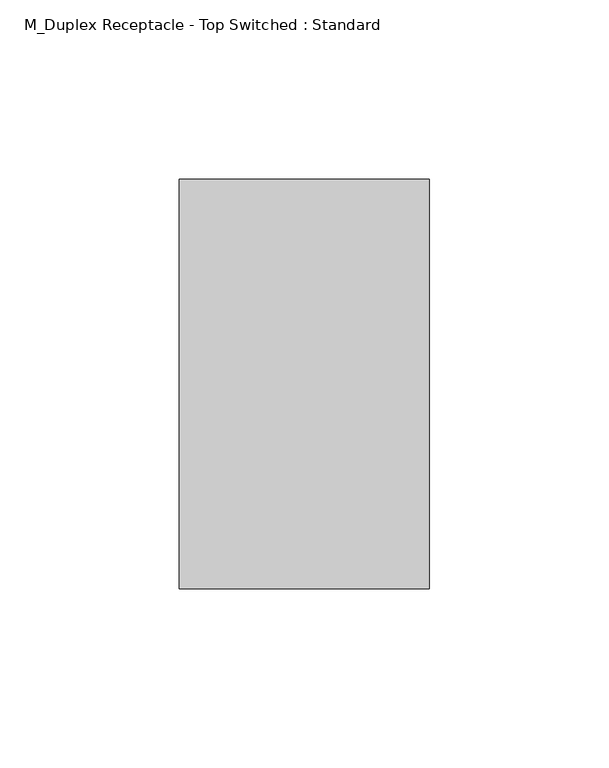
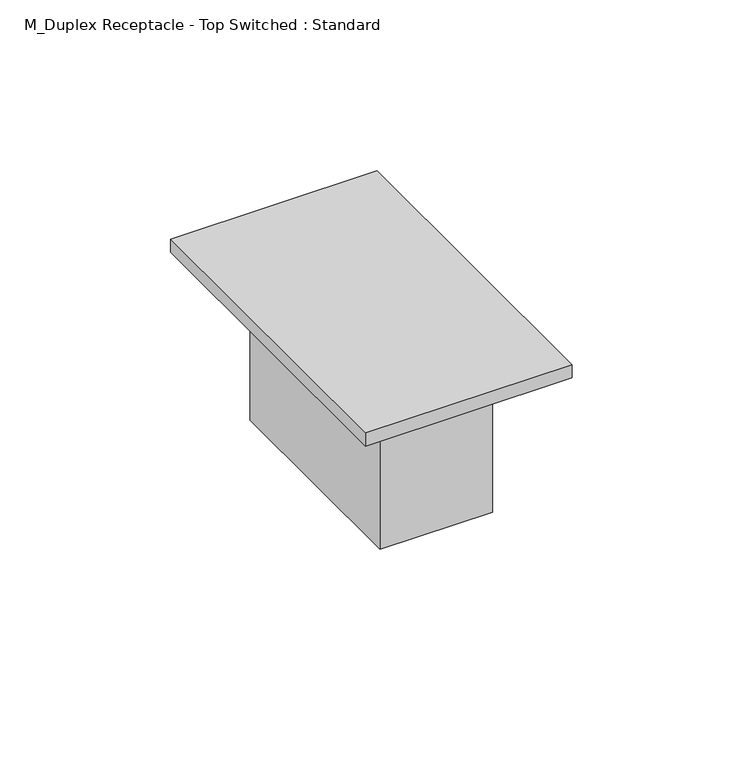
"""IFC4 building model written with IfcOpenShell, lengths in millimetres: proxy geometry, M_Duplex Receptacle - Top Switched : Standard."""

from ifc_helpers import new_model, si_unit, frame, origin, origin_with_axes, place, context, project, spatial, polyline, outline, extrude, source, transform, mapped, element, save


def m_duplex_receptacle_top_switched_standard_10251bba(model_context):
    return source(origin(), model_context, "Body", "SweptSolid", [
        extrude(outline(polyline([(19.05, 38.1), (19.05, -38.1), (-19.05, -38.1), (-19.05, 38.1), (19.05, 38.1)])), frame((0.0, 0.0, -53.975), z_axis=(0.0, 0.0, 1.0), x_axis=(1.0, 0.0, 0.0)), (0.0, 0.0, 1.0), 53.975),
        extrude(outline(polyline([(34.925, 57.15), (34.925, -57.15), (-34.925, -57.15), (-34.925, 57.15), (34.925, 57.15)])), origin_with_axes(), (0.0, 0.0, 1.0), 4.7625),
    ])


if __name__ == "__main__":
    model = new_model("IFC4")
    model_context = context("Model", 3, world=origin())
    ifc_project = project(units=[si_unit("LENGTHUNIT", "METRE", prefix="MILLI")], contexts=[model_context])
    site = spatial("IfcSite", under=ifc_project)
    building = spatial("IfcBuilding", under=site)
    placement = place(None, origin())
    m_duplex_receptacle_top_switched_standard_shape = m_duplex_receptacle_top_switched_standard_10251bba(model_context)
    element("IfcBuildingElementProxy", 1, Name="M_Duplex Receptacle - Top Switched : Standard", ObjectType="M_Duplex Receptacle - Top Switched : Standard", at=placement, inside=building, context=model_context, shape_type="MappedRepresentation", body=[
        mapped(m_duplex_receptacle_top_switched_standard_shape, transform((0.0, 0.0, 0.0), x_axis=(1.0, 0.0, 0.0), y_axis=(0.0, 1.0, 0.0), z_axis=(0.0, 0.0, 1.0))),
    ])
    save(model, "model.ifc")

# Revit data of these elements
# Type "M_Duplex Receptacle - Top Switched : Standard"
#   Type Mark = "M_Duplex Receptacle - Top Switched"
#   Classification.OmniClass.21.Number = "21-04 50 30 50"
#   Classification.MasterFormat.Description = "Wiring Devices"
#   Classification.OmniClass.22.Number = "22-26 27 26"
#   Classification.OmniClass.21.Description = "Wiring Devices"
#   Classification.UniFormat.II.Description = "Wiring Devices"
#   Classification.MasterFormat.Number = "26 27 26"
#   Classification.OmniClass.23.Number = "23-35 27 11"
#   Classification.OmniClass.22.Description = "Wiring Devices"
#   Classification.OmniClass.23.Description = "Electrical Receptacles"
#   Classification.UniFormat.II.Number = "D5030.50"
#   COBie.Type.CreatedBy = "info@mma.ie"
#   COBie.Type.CreatedOn = "2017-07-25T10:15:16"
#   COBie.Type.Name = "M_Duplex Receptacle - Top Switched"
#   COBie.Type.Category = "23-35 27 11 : Electrical Receptacles"
#   COBie.Type.Description = "M_Duplex Receptacle - Top Switched_Standard"
#   COBie.Type.AssetType = "Fixed"
#   COBie.Type.Manufacturer = ""
#   COBie.Type.ModelNumber = ""
#   Keynote = "26 27 26.B"
#   COBie.Type.ReplacementCost = 0
#   Switch Voltage = 220 V
#   Recep.Width = 69.85 mm
#   Recep.Load = 180 VA
#   Recep.Height = 114.3 mm
#   Load = 180 VA
#   Default Elevation = 460 mm
#   COBie.Type = yes
#   Recep.Material = Stainless Steel
#   Load Classification = Receptacle
#   Assembly Code = ""
# Materials
#   "Stainless Steel": class "Metal", colour RGB 120 120 120, transparency 0, Description = "Stainless Steel 18/8", Cost = 0
